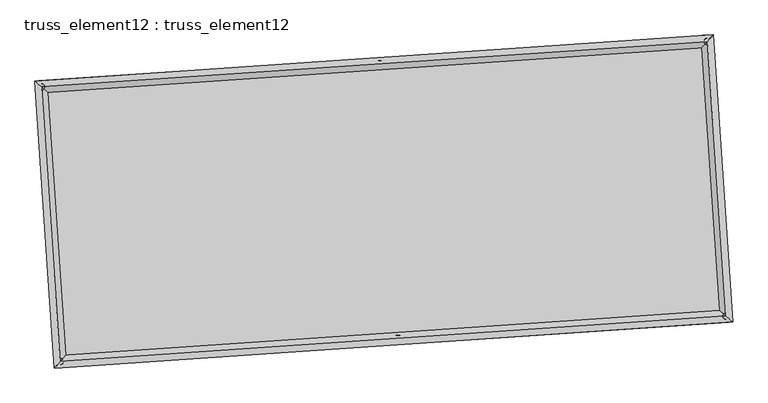
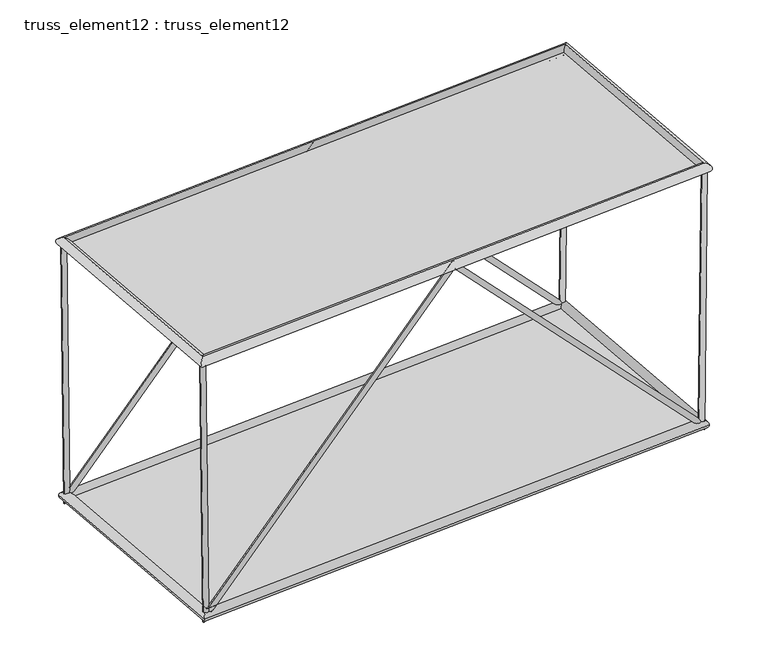
"""IFC4 building model written with IfcOpenShell, lengths in millimetres: plate geometry, truss_element12 : truss_element12."""

import ifcopenshell
import ifcopenshell.guid

model = None  # the IFC model being written
_history = None  # IfcOwnerHistory: only IFC2X3 demands one
_inside = {}  # id of a spatial element -> (the spatial element, [elements in it])
_under = {}  # id of a project, library or spatial element -> (it, [spatial elements below it])
_declared = {}  # id of a project -> (the project, [libraries it declares])
_typed = {}  # id of a type object -> (the type object, [elements of that type])
_made_of = {}  # id of a material, layer set ... -> (it, [elements and type objects made of it])


def new_model(schema):
    """Start an empty IFC model of exactly this schema.

    Asked for "IFC4X3", IfcOpenShell would pick the latest addendum, in which some entities
    have other attributes; the version numbers below select the first issue.
    IFC2X3 requires an IfcOwnerHistory on every rooted entity: one is made here for all.
    """
    global model, _history
    if schema == "IFC4X3":
        model = ifcopenshell.file(schema_version=(4, 3, 0, 0))
    else:
        model = ifcopenshell.file(schema=schema)
    _inside.clear()
    _under.clear()
    _declared.clear()
    _typed.clear()
    _made_of.clear()
    _history = None
    if model.schema == "IFC2X3":
        org = make("IfcOrganization", Name="unknown")
        user = make(
            "IfcPersonAndOrganization",
            ThePerson=make("IfcPerson", FamilyName="unknown"),
            TheOrganization=org,
        )
        app = make(
            "IfcApplication",
            ApplicationDeveloper=org,
            Version="unknown",
            ApplicationFullName="unknown",
            ApplicationIdentifier="unknown",
        )
        _history = make(
            "IfcOwnerHistory",
            OwningUser=user,
            OwningApplication=app,
            ChangeAction="ADDED",
            CreationDate=0,
        )
    return model


def make(cls, **values):
    """One entity of the class cls with the attributes given. An attribute that is None is left unset."""
    return model.create_entity(
        cls, **{name: value for name, value in values.items() if value is not None}
    )


def rooted(cls, **values):
    """An entity with a GlobalId (a new one), such as an element, a storey or a relation."""
    return make(cls, GlobalId=ifcopenshell.guid.new(), OwnerHistory=_history, **values)


def si_unit(unit_type, name, prefix=None):
    """IfcSIUnit, for example si_unit("LENGTHUNIT", "METRE", prefix="MILLI")."""
    return make("IfcSIUnit", UnitType=unit_type, Prefix=prefix, Name=name)


def assignment(units):
    """IfcUnitAssignment: the units of a project."""
    return None if units is None else make("IfcUnitAssignment", Units=units)


def point(xyz):
    """IfcCartesianPoint."""
    return None if xyz is None else make("IfcCartesianPoint", Coordinates=xyz)


def direction(xyz):
    """IfcDirection."""
    return None if xyz is None else make("IfcDirection", DirectionRatios=xyz)


def frame(location, z_axis=None, x_axis=None):
    """IfcAxis2Placement3D, a coordinate frame: its origin and axes. An axis left out is left unset."""
    return make(
        "IfcAxis2Placement3D",
        Location=point(location),
        Axis=direction(z_axis),
        RefDirection=direction(x_axis),
    )


def origin():
    """The frame at (0, 0, 0) with its axes left unset."""
    return frame((0.0, 0.0, 0.0))


def origin_with_axes():
    """The frame at (0, 0, 0) with the z axis (0, 0, 1) and the x axis (1, 0, 0) written out."""
    return frame((0.0, 0.0, 0.0), z_axis=(0.0, 0.0, 1.0), x_axis=(1.0, 0.0, 0.0))


def place(relative_to, where):
    """IfcLocalPlacement: puts the frame where relative to a parent placement (None: the world)."""
    return make(
        "IfcLocalPlacement", PlacementRelTo=relative_to, RelativePlacement=where
    )


def context(
    kind, dimensions, precision=None, world=None, true_north=None, identifier=None
):
    """IfcGeometricRepresentationContext, for example the 3D "Model" context."""
    return make(
        "IfcGeometricRepresentationContext",
        ContextIdentifier=identifier,
        ContextType=kind,
        CoordinateSpaceDimension=dimensions,
        Precision=precision,
        WorldCoordinateSystem=world,
        TrueNorth=true_north,
    )


def project(units=None, contexts=None):
    """IfcProject with its units and contexts."""
    return rooted(
        "IfcProject",
        Name="project",
        RepresentationContexts=contexts,
        UnitsInContext=assignment(units),
    )


def spatial(cls, under=None, at=None, **own):
    """A site, building, storey or space (cls), placed at a placement, below another one or the project."""
    s = rooted(cls, ObjectPlacement=at, **own)
    if under is not None:
        _under.setdefault(under.id(), (under, []))[1].append(s)
    return s


def polyline(points):
    """IfcPolyline through the points."""
    return make("IfcPolyline", Points=[point(p) for p in points])


def circle_curve(where, radius):
    """IfcCircle in the frame where."""
    return make("IfcCircle", Position=where, Radius=radius)


def ellipse_curve(where, semi_axis1, semi_axis2):
    """IfcEllipse in the frame where."""
    return make(
        "IfcEllipse", Position=where, SemiAxis1=semi_axis1, SemiAxis2=semi_axis2
    )


def outline(outer, holes=None, kind="AREA"):
    """IfcArbitraryClosedProfileDef: a profile drawn as a closed curve; with holes, ...WithVoids."""
    if holes is None:
        return make("IfcArbitraryClosedProfileDef", ProfileType=kind, OuterCurve=outer)
    return make(
        "IfcArbitraryProfileDefWithVoids",
        ProfileType=kind,
        OuterCurve=outer,
        InnerCurves=holes,
    )


def extrude(swept, where, along, depth):
    """IfcExtrudedAreaSolid: the profile swept, set in the frame where, extruded along a direction by depth."""
    return make(
        "IfcExtrudedAreaSolid",
        SweptArea=swept,
        Position=where,
        ExtrudedDirection=direction(along),
        Depth=depth,
    )


def shape(context_of_items, identifier, shape_type, items):
    """IfcShapeRepresentation: the items that make up one representation, for example the "Body"."""
    return make(
        "IfcShapeRepresentation",
        ContextOfItems=context_of_items,
        RepresentationIdentifier=identifier,
        RepresentationType=shape_type,
        Items=items,
    )


def source(mapping_origin, context_of_items, identifier, shape_type, items):
    """IfcRepresentationMap: a shape defined once, which mapped items show again and again."""
    return make(
        "IfcRepresentationMap",
        MappingOrigin=mapping_origin,
        MappedRepresentation=shape(context_of_items, identifier, shape_type, items),
    )


def transform(
    local_origin,
    x_axis=None,
    y_axis=None,
    z_axis=None,
    scale=None,
    scale2=None,
    scale3=None,
    uniform=True,
):
    """IfcCartesianTransformationOperator3D, or its non-uniform kind. x_axis, y_axis, z_axis: its Axis1, 2, 3."""
    if uniform:
        return make(
            "IfcCartesianTransformationOperator3D",
            Axis1=direction(x_axis),
            Axis2=direction(y_axis),
            LocalOrigin=point(local_origin),
            Scale=scale,
            Axis3=direction(z_axis),
        )
    return make(
        "IfcCartesianTransformationOperator3DnonUniform",
        Axis1=direction(x_axis),
        Axis2=direction(y_axis),
        LocalOrigin=point(local_origin),
        Scale=scale,
        Axis3=direction(z_axis),
        Scale2=scale2,
        Scale3=scale3,
    )


def mapped(mapping_source, mapping_target):
    """IfcMappedItem: shows the shape of a source again, moved by a transform."""
    return make(
        "IfcMappedItem", MappingSource=mapping_source, MappingTarget=mapping_target
    )


def made_of(thing, what):
    """Note that an element or type object is made of a material, layer set ...; save() writes the relation."""
    if what is not None:
        _made_of.setdefault(what.id(), (what, []))[1].append(thing)
    return thing


def element(
    cls,
    number,
    at=None,
    inside=None,
    cuts=None,
    type_object=None,
    material=None,
    context=None,
    identifier="Body",
    shape_type=None,
    held_by="IfcProductDefinitionShape",
    body=None,
    shapes=None,
    **own,
):
    """One element of the class cls, such as IfcWall. Its Tag is "e" and its number.

    at: its placement. inside: the storey or other place that contains it. cuts: it is an
    opening in that element (IfcRelVoidsElement). A single representation is given by context,
    identifier, shape_type and body (its items); several are given by shapes. held_by: the class
    of the entity that holds the representations. save() writes the other relations.
    """
    e = rooted(cls, Tag="e%d" % number, ObjectPlacement=at, **own)
    if body is not None:
        shapes = [shape(context, identifier, shape_type, body)]
    if shapes is not None:
        e.Representation = make(held_by, Representations=shapes)
    if inside is not None:
        _inside.setdefault(inside.id(), (inside, []))[1].append(e)
    if cuts is not None:
        rooted(
            "IfcRelVoidsElement", RelatingBuildingElement=cuts, RelatedOpeningElement=e
        )
    if type_object is not None:
        _typed.setdefault(type_object.id(), (type_object, []))[1].append(e)
    return made_of(e, material)


def aggregate(whole, parts):
    """IfcRelAggregates: a whole, such as a stair, and the parts it consists of."""
    return rooted("IfcRelAggregates", RelatingObject=whole, RelatedObjects=parts)


def save(model, path):
    """Write the relations noted so far, then the file.

    IfcRelAggregates (storeys below a building ...), IfcRelContainedInSpatialStructure (elements
    in a storey), IfcRelDefinesByType, IfcRelAssociatesMaterial and IfcRelDeclares: one each for
    every whole, place, type object, material and project.
    """
    for whole, parts in _under.values():
        aggregate(whole, parts)
    for where, things in _inside.values():
        rooted(
            "IfcRelContainedInSpatialStructure",
            RelatedElements=things,
            RelatingStructure=where,
        )
    for kind, things in _typed.values():
        rooted("IfcRelDefinesByType", RelatedObjects=things, RelatingType=kind)
    for what, things in _made_of.values():
        rooted("IfcRelAssociatesMaterial", RelatedObjects=things, RelatingMaterial=what)
    for by, libraries in _declared.values():
        rooted("IfcRelDeclares", RelatingContext=by, RelatedDefinitions=libraries)
    model.write(path)


def plane_surface(at):
    """IfcPlane: the flat surface through the origin of the frame at, square to its z axis."""
    return make("IfcPlane", Position=at)


def cylinder_surface(at, radius):
    """IfcCylindricalSurface: all points at the distance radius from the z axis of the frame at."""
    return make("IfcCylindricalSurface", Position=at, Radius=radius)


def advanced_brep(points, edges, surfaces, faces):
    """IfcAdvancedBrep: a solid bounded by faces that lie on surfaces and meet in shared edges.

    An edge is (start, end): straight between two places in points (the first is 0);
    or (start, end, curve); or (start, end, curve, False) where it runs against its curve.
    A face is (place in surfaces, loops), or (place, loops, False) where it looks against
    its surface's normal. A loop lists edges by number (the first is 1), with a minus sign
    where the edge is run from its end to its start. The first loop is the outer one.
    """
    corners = [point(p) for p in points]
    vertices = [make("IfcVertexPoint", VertexGeometry=c) for c in corners]
    made = []
    for start, end, *more in edges:
        made.append(
            make(
                "IfcEdgeCurve",
                EdgeStart=vertices[start],
                EdgeEnd=vertices[end],
                EdgeGeometry=more[0] if more else make("IfcPolyline", Points=[corners[start], corners[end]]),
                SameSense=more[1] if len(more) > 1 else True,
            )
        )
    hull = []
    for where, loops, *sense in faces:
        bounds = []
        for j, loop in enumerate(loops):
            ring = [make("IfcOrientedEdge", EdgeElement=made[abs(k) - 1], Orientation=k > 0) for k in loop]
            bounds.append(
                make(
                    "IfcFaceOuterBound" if j == 0 else "IfcFaceBound",
                    Bound=make("IfcEdgeLoop", EdgeList=ring),
                    Orientation=True,
                )
            )
        hull.append(make("IfcAdvancedFace", Bounds=bounds, FaceSurface=surfaces[where], SameSense=sense[0] if sense else True))
    return make("IfcAdvancedBrep", Outer=make("IfcClosedShell", CfsFaces=hull))


def truss_element12_truss_element12_1e288aef(model_context):
    return source(origin(), model_context, "Body", "SolidModel", [
        advanced_brep(
        [(-3721.8541699, 2272.3433372, 5000.243792), (-3820.9510531, 2258.982503, 4999.1054445), (-3666.3357635, 2276.1289263, 122.7527544), (-3762.6511193, 2262.9577538, -122.7527544), (1063.2103796, 2598.6186991, 5071.8018953), (1063.6661844, 2592.0459842, 4927.5587941), (5793.7499875, 2921.1762125, 122.759853), (5891.0109895, 2921.204276, -122.759853), (5848.2824161, 2924.8945715, 5000.2451385), (5948.275935, 2925.108955, 4999.1270036)],
        [
            (0, 1, circle_curve(frame((-3771.4026115, 2265.6629201, 4999.6746183), z_axis=(-0.011381834017515616, -0.0007760839952527173, 0.9999349236565499), x_axis=(-0.13360848187270624, 0.9910339089151396, -0.0007516329220677924)), 50.0)),
            (1, 0, circle_curve(frame((-3771.4026115, 2265.6629201, 4999.6746183), z_axis=(-0.011381834017515616, -0.0007760839952527173, 0.9999349236565499), x_axis=(-0.13360848187270624, 0.9910339089151396, -0.0007516329220677924)), 50.0)),
            (0, 2),
            (2, 3, ellipse_curve(frame((-3714.4934414, 2269.54334, 0.0), z_axis=(-0.9278994784854547, -0.06326993816178475, 0.36742274392234436), x_axis=(0.36657157095159426, 0.024995121954192616, 0.9300540453374608)), 132.271936, 50.0)),
            (3, 1),
            (3, 2, ellipse_curve(frame((-3714.4934414, 2269.54334, 0.0), z_axis=(-0.9278994784854547, -0.06326993816178475, 0.36742274392234436), x_axis=(0.36657157095159426, 0.024995121954192616, 0.9300540453374608)), 132.271936, 50.0)),
            (2, 4),
            (4, 5, ellipse_curve(frame((1063.438282, 2595.3323417, 4999.6803447), z_axis=(-0.9976833946832313, -0.06802823813381093, -5.281811364997211e-05), x_axis=(5.2695755000598474e-05, 3.593123218122507e-06, -0.9999999986051235)), 72.2785958, 50.0)),
            (5, 3),
            (5, 4, ellipse_curve(frame((1063.438282, 2595.3323417, 4999.6803447), z_axis=(-0.9976833946832313, -0.06802823813381093, -5.281811364997211e-05), x_axis=(5.2695755000598474e-05, 3.593123218122507e-06, -0.9999999986051235)), 72.2785958, 50.0)),
            (4, 6),
            (6, 7, ellipse_curve(frame((5842.3804885, 2921.1902443, 0.0), z_axis=(-0.9278429760300568, -0.06326608547413708, -0.3675660678850353), x_axis=(-0.3667145628894308, -0.025004872030870366, 0.9299974116843194)), 132.2876405, 50.0)),
            (7, 5),
            (7, 6, ellipse_curve(frame((5842.3804885, 2921.1902443, 0.0), z_axis=(-0.9278429760300568, -0.06326608547413708, -0.3675660678850353), x_axis=(-0.3667145628894308, -0.025004872030870366, 0.9299974116843194)), 132.2876405, 50.0)),
            (8, 9, circle_curve(frame((5898.2791756, 2925.0017632, 4999.6860711), z_axis=(0.011179737411862272, 0.0007623037959543959, 0.9999372142111346), x_axis=(-0.002152223979418104, 0.9999974114288641, -0.0007382868776594081)), 50.0)),
            (9, 8, circle_curve(frame((5898.2791756, 2925.0017632, 4999.6860711), z_axis=(0.011179737411862272, 0.0007623037959543959, 0.9999372142111346), x_axis=(-0.002152223979418104, 0.9999974114288641, -0.0007382868776594081)), 50.0)),
            (6, 8),
            (9, 7),
        ],
        [
            plane_surface(frame((-3771.4026115, 2315.662905, 4999.713425), z_axis=(-0.01138183401751662, -0.0007760839952526837, 0.99993492365655), x_axis=(0.9999352248292876, -8.833831430798961e-06, 0.01138183058939645))),
            cylinder_surface(frame((-3771.4026115, 2265.6629201, 4999.6746183), z_axis=(-0.011381834017515616, -0.0007760839952527173, 0.9999349236565499), x_axis=(-0.13360848187270624, 0.9910339089151396, -0.0007516329220677924)), 50.0),
            cylinder_surface(frame((-3714.4934414, 2269.54334, 0.0), z_axis=(-0.6901271226391988, -0.04705714507397151, -0.7221566171511742), x_axis=(-0.0204113902098155, 0.9987523882932022, -0.045574576556754245)), 50.0),
            cylinder_surface(frame((1063.438282, 2595.3323417, 4999.6803447), z_axis=(-0.690203227964863, -0.04706233440682505, 0.72208354141821), x_axis=(-0.11534466276751382, 0.9922792493126465, -0.04557960239601923)), 50.0),
            plane_surface(frame((5898.2791756, 2875.0017778, 4999.7241886), z_axis=(0.011179737411861788, 0.0007623037959489832, 0.9999372142111346), x_axis=(0.9999375047828748, -8.522888906625786e-06, -0.011179734163143003))),
            cylinder_surface(frame((5842.3804885, 2921.1902443, 0.0), z_axis=(-0.011179737411862274, -0.0007623037959543961, -0.9999372142111348), x_axis=(-0.002152223979418104, 0.9999974114288641, -0.0007382868776594081)), 50.0),
        ],
        [
            (0, [[1, 2]]),
            (1, [[-1, 3, 4, 5]]),
            (1, [[-2, -5, 6, -3]]),
            (2, [[-4, 7, 8, 9]]),
            (2, [[-6, -9, 10, -7]]),
            (3, [[-8, 11, 12, 13]]),
            (3, [[-10, -13, 14, -11]]),
            (4, [[15, 16]]),
            (5, [[-12, 17, -16, 18]]),
            (5, [[-14, -18, -15, -17]]),
        ],
    ),
        advanced_brep(
        [(-3449.741217, -1718.3902471, 5000.243792), (-3548.8381002, -1731.7510813, 4999.1054445), (-3394.2228106, -1714.604658, 122.7527544), (-3490.5381664, -1727.7758305, -122.7527544), (1335.3233326, -1392.1148852, 5071.8018953), (1335.7791373, -1398.6876001, 4927.5587941), (6065.8629405, -1069.5573718, 122.759853), (6163.1239424, -1069.5293083, -122.759853), (6120.395369, -1065.8390128, 5000.2451385), (6220.3888879, -1065.6246293, 4999.1270036)],
        [
            (0, 1, circle_curve(frame((-3499.2896586, -1725.0706642, 4999.6746183), z_axis=(-0.0113818340175155, -0.0007760839952527034, 0.9999349236565499), x_axis=(-0.1336084818727064, 0.9910339089151396, -0.0007516329220677924)), 50.0)),
            (1, 0, circle_curve(frame((-3499.2896586, -1725.0706642, 4999.6746183), z_axis=(-0.0113818340175155, -0.0007760839952527034, 0.9999349236565499), x_axis=(-0.1336084818727064, 0.9910339089151396, -0.0007516329220677924)), 50.0)),
            (0, 2),
            (2, 3, ellipse_curve(frame((-3442.3804885, -1721.1902443, 0.0), z_axis=(-0.927899478485455, -0.06326993816178478, 0.3674227439223443), x_axis=(0.36657157095159415, 0.02499512195419262, 0.9300540453374606)), 132.271936, 50.0)),
            (3, 1),
            (3, 2, ellipse_curve(frame((-3442.3804885, -1721.1902443, 0.0), z_axis=(-0.927899478485455, -0.06326993816178478, 0.3674227439223443), x_axis=(0.36657157095159415, 0.02499512195419262, 0.9300540453374606)), 132.271936, 50.0)),
            (2, 4),
            (4, 5, ellipse_curve(frame((1335.5512349, -1395.4012426, 4999.6803447), z_axis=(-0.9976833946832313, -0.06802823813381102, -5.281811365021285e-05), x_axis=(5.269575500075221e-05, 3.59312321818977e-06, -0.9999999986051235)), 72.2785958, 50.0)),
            (5, 3),
            (5, 4, ellipse_curve(frame((1335.5512349, -1395.4012426, 4999.6803447), z_axis=(-0.9976833946832313, -0.06802823813381102, -5.281811365021285e-05), x_axis=(5.269575500075221e-05, 3.59312321818977e-06, -0.9999999986051235)), 72.2785958, 50.0)),
            (4, 6),
            (6, 7, ellipse_curve(frame((6114.4934414, -1069.54334, 0.0), z_axis=(-0.9278429760300566, -0.06326608547413719, -0.36756606788503576), x_axis=(-0.3667145628894313, -0.025004872030870456, 0.9299974116843193)), 132.2876405, 50.0)),
            (7, 5),
            (7, 6, ellipse_curve(frame((6114.4934414, -1069.54334, 0.0), z_axis=(-0.9278429760300566, -0.06326608547413719, -0.36756606788503576), x_axis=(-0.3667145628894313, -0.025004872030870456, 0.9299974116843193)), 132.2876405, 50.0)),
            (8, 9, circle_curve(frame((6170.3921285, -1065.7318211, 4999.6860711), z_axis=(0.011179737411862045, 0.0007623037959543686, 0.9999372142111348), x_axis=(-0.0021522239794181794, 0.999997411428864, -0.0007382868776593801)), 50.0)),
            (9, 8, circle_curve(frame((6170.3921285, -1065.7318211, 4999.6860711), z_axis=(0.011179737411862045, 0.0007623037959543686, 0.9999372142111348), x_axis=(-0.0021522239794181794, 0.999997411428864, -0.0007382868776593801)), 50.0)),
            (6, 8),
            (9, 7),
        ],
        [
            plane_surface(frame((-3499.2896586, -1675.0706793, 4999.713425), z_axis=(-0.01138183401751662, -0.0007760839952526816, 0.99993492365655), x_axis=(0.9999352248292876, -8.833831430798961e-06, 0.01138183058939645))),
            cylinder_surface(frame((-3499.2896586, -1725.0706642, 4999.6746183), z_axis=(-0.0113818340175155, -0.0007760839952527034, 0.9999349236565499), x_axis=(-0.1336084818727064, 0.9910339089151396, -0.0007516329220677924)), 50.0),
            cylinder_surface(frame((-3442.3804885, -1721.1902443, 0.0), z_axis=(-0.6901271226391986, -0.04705714507397152, -0.7221566171511744), x_axis=(-0.020411390209815434, 0.9987523882932022, -0.045574576556754315)), 50.0),
            cylinder_surface(frame((1335.5512349, -1395.4012426, 4999.6803447), z_axis=(-0.6902032279648631, -0.047062334406825154, 0.7220835414182099), x_axis=(-0.11534466276751408, 0.9922792493126465, -0.04557960239601936)), 50.0),
            plane_surface(frame((6170.3921285, -1115.7318065, 4999.7241886), z_axis=(0.011179737411861788, 0.0007623037959489812, 0.9999372142111346), x_axis=(0.9999375047828748, -8.522888906625786e-06, -0.011179734163143003))),
            cylinder_surface(frame((6114.4934414, -1069.54334, 0.0), z_axis=(-0.011179737411862043, -0.0007623037959543684, -0.9999372142111346), x_axis=(-0.0021522239794181794, 0.999997411428864, -0.0007382868776593801)), 50.0),
        ],
        [
            (0, [[1, 2]]),
            (1, [[-1, 3, 4, 5]]),
            (1, [[-2, -5, 6, -3]]),
            (2, [[-4, 7, 8, 9]]),
            (2, [[-6, -9, 10, -7]]),
            (3, [[-8, 11, 12, 13]]),
            (3, [[-10, -13, 14, -11]]),
            (4, [[15, 16]]),
            (5, [[-12, 17, -16, 18]]),
            (5, [[-14, -18, -15, -17]]),
        ],
    ),
        advanced_brep(
        [(-3499.2866492, -1725.0673288, 4909.6746183), (-3499.292668, -1725.0739997, 5089.6746182), (-3771.4060458, 2265.6658161, 5089.6746182), (-3771.3991772, 2265.660024, 4909.6746183), (5898.2819728, 2925.0050842, 5089.686071), (5898.2763784, 2924.9984423, 4909.6860711), (6170.3953506, -1065.7347316, 5089.686071), (6170.3889064, -1065.7289105, 4909.6860711)],
        [
            (0, 1, ellipse_curve(frame((-3499.2896586, -1725.0706642, 4999.6746183), z_axis=(-0.7535719234049658, 0.657365466278114, -8.3555725473804e-07), x_axis=(-0.6573654662775879, -0.7535719234054246, -8.355572547380254e-07)), 127.2792206, 90.0)),
            (1, 2),
            (2, 3, ellipse_curve(frame((-3771.4026115, 2265.6629201, 4999.6746183), z_axis=(-0.6573654662775877, -0.7535719234054249, -8.355572547380119e-07), x_axis=(0.7535719234049659, -0.6573654662781139, 8.355572547380267e-07)), 127.2792206, 90.0)),
            (3, 0),
            (1, 0, ellipse_curve(frame((-3499.2896586, -1725.0706642, 4999.6746183), z_axis=(-0.7535719234049658, 0.657365466278114, -8.3555725473804e-07), x_axis=(-0.6573654662775879, -0.7535719234054246, -8.355572547380254e-07)), 127.2792206, 90.0)),
            (3, 2, ellipse_curve(frame((-3771.4026115, 2265.6629201, 4999.6746183), z_axis=(-0.6573654662775877, -0.7535719234054249, -8.355572547380119e-07), x_axis=(0.7535719234049659, -0.6573654662781139, 8.355572547380267e-07)), 127.2792206, 90.0)),
            (2, 4),
            (4, 5, ellipse_curve(frame((5898.2791756, 2925.0017632, 4999.6860711), z_axis=(-0.7535719234049658, 0.657365466278114, -8.355572547380136e-07), x_axis=(-0.6573654662775879, -0.7535719234054248, -8.355572547380251e-07)), 127.2792206, 90.0)),
            (5, 3),
            (5, 4, ellipse_curve(frame((5898.2791756, 2925.0017632, 4999.6860711), z_axis=(-0.7535719234049658, 0.657365466278114, -8.355572547380136e-07), x_axis=(-0.6573654662775879, -0.7535719234054248, -8.355572547380251e-07)), 127.2792206, 90.0)),
            (4, 6),
            (6, 7, ellipse_curve(frame((6170.3921285, -1065.7318211, 4999.6860711), z_axis=(0.6573654662775877, 0.7535719234054248, 8.355572547380384e-07), x_axis=(-0.7535719234049659, 0.657365466278114, -8.355572547380273e-07)), 127.2792206, 90.0)),
            (7, 5),
            (7, 6, ellipse_curve(frame((6170.3921285, -1065.7318211, 4999.6860711), z_axis=(0.6573654662775877, 0.7535719234054248, 8.355572547380384e-07), x_axis=(-0.7535719234049659, 0.657365466278114, -8.355572547380273e-07)), 127.2792206, 90.0)),
            (6, 1),
            (0, 7),
        ],
        [
            cylinder_surface(frame((-3499.2896586, -1725.0706642, 4999.6746183), z_axis=(0.06802823822870131, -0.9976833960748765, 0.0), x_axis=(-0.9976833954326236, -0.06802823818490852, -3.58815903472379e-05)), 90.0),
            cylinder_surface(frame((-3771.4026115, 2265.6629201, 4999.6746183), z_axis=(-0.99768339607418, -0.06802823822865506, -1.1816564017897381e-06), x_axis=(-0.06802823814683823, 0.9976833954770179, -3.4699933946159566e-05)), 90.0),
            cylinder_surface(frame((5898.2791756, 2925.0017632, 4999.6860711), z_axis=(-0.06802823822870106, 0.9976833960748765, 0.0), x_axis=(0.9976833955144404, 0.06802823819048705, -3.351827754508122e-05)), 90.0),
            cylinder_surface(frame((6170.3921285, -1065.7318211, 4999.6860711), z_axis=(0.99768339607418, 0.06802823822865493, 1.181656401789757e-06), x_axis=(0.06802823822865493, -0.9976833954714391, -3.469993394615955e-05)), 90.0),
        ],
        [
            (0, [[1, 2, 3, 4]]),
            (0, [[5, -4, 6, -2]]),
            (1, [[-3, 7, 8, 9]]),
            (1, [[-6, -9, 10, -7]]),
            (2, [[-8, 11, 12, 13]]),
            (2, [[-10, -13, 14, -11]]),
            (3, [[-12, 15, -1, 16]]),
            (3, [[-14, -16, -5, -15]]),
        ],
    ),
        advanced_brep(
        [(-3358.7115243, -1625.2761972, 0.0), (-3526.0494527, -1817.1042913, 0.0), (-3810.4074885, 2353.2123043, 0.0), (-3618.5793943, 2185.8743758, 0.0), (5926.0494527, 3017.1042913, 0.0), (5758.7115243, 2825.2761972, 0.0), (6210.4074885, -1153.2123043, 0.0), (6018.5793943, -985.8743758, 0.0)],
        [
            (0, 1, ellipse_curve(frame((-3442.3804885, -1721.1902443, 0.0), z_axis=(-0.7535719234054579, 0.6573654662780809, 0.0), x_axis=(-0.657365466278081, -0.7535719234054578, 0.0)), 127.2792206, 90.0)),
            (1, 2),
            (2, 3, ellipse_curve(frame((-3714.4934414, 2269.54334, 0.0), z_axis=(-0.6573654662780808, -0.7535719234054579, 0.0), x_axis=(0.7535719234054578, -0.6573654662780809, 0.0)), 127.2792206, 90.0)),
            (3, 0),
            (1, 0, ellipse_curve(frame((-3442.3804885, -1721.1902443, 0.0), z_axis=(-0.7535719234054579, 0.6573654662780809, 0.0), x_axis=(-0.657365466278081, -0.7535719234054578, 0.0)), 127.2792206, 90.0)),
            (3, 2, ellipse_curve(frame((-3714.4934414, 2269.54334, 0.0), z_axis=(-0.6573654662780808, -0.7535719234054579, 0.0), x_axis=(0.7535719234054578, -0.6573654662780809, 0.0)), 127.2792206, 90.0)),
            (2, 4),
            (4, 5, ellipse_curve(frame((5842.3804885, 2921.1902443, 0.0), z_axis=(-0.7535719234054579, 0.6573654662780809, 0.0), x_axis=(-0.6573654662780809, -0.7535719234054578, 0.0)), 127.2792206, 90.0)),
            (5, 3),
            (5, 4, ellipse_curve(frame((5842.3804885, 2921.1902443, 0.0), z_axis=(-0.7535719234054579, 0.6573654662780809, 0.0), x_axis=(-0.6573654662780809, -0.7535719234054578, 0.0)), 127.2792206, 90.0)),
            (4, 6),
            (6, 7, ellipse_curve(frame((6114.4934414, -1069.54334, 0.0), z_axis=(0.6573654662780809, 0.7535719234054579, 0.0), x_axis=(-0.7535719234054578, 0.6573654662780809, 0.0)), 127.2792206, 90.0)),
            (7, 5),
            (7, 6, ellipse_curve(frame((6114.4934414, -1069.54334, 0.0), z_axis=(0.6573654662780809, 0.7535719234054579, 0.0), x_axis=(-0.7535719234054578, 0.6573654662780809, 0.0)), 127.2792206, 90.0)),
            (6, 1),
            (0, 7),
        ],
        [
            cylinder_surface(frame((-3442.3804885, -1721.1902443, 0.0), z_axis=(0.06802823822870059, -0.9976833960748767, 0.0), x_axis=(-0.9976833960748767, -0.06802823822870059, 0.0)), 90.0),
            cylinder_surface(frame((-3714.4934414, 2269.54334, 0.0), z_axis=(-0.9976833960748767, -0.06802823822870172, 0.0), x_axis=(-0.06802823822870172, 0.9976833960748767, 0.0)), 90.0),
            cylinder_surface(frame((5842.3804885, 2921.1902443, 0.0), z_axis=(-0.06802823822870048, 0.9976833960748768, 0.0), x_axis=(0.9976833960748768, 0.06802823822870048, 0.0)), 90.0),
            cylinder_surface(frame((6114.4934414, -1069.54334, 0.0), z_axis=(0.9976833960748767, 0.06802823822870152, 0.0), x_axis=(0.06802823822870152, -0.9976833960748767, 0.0)), 90.0),
        ],
        [
            (0, [[1, 2, 3, 4]]),
            (0, [[5, -4, 6, -2]]),
            (1, [[-3, 7, 8, 9]]),
            (1, [[-6, -9, 10, -7]]),
            (2, [[-8, 11, 12, 13]]),
            (2, [[-10, -13, 14, -11]]),
            (3, [[-12, 15, -1, 16]]),
            (3, [[-14, -16, -5, -15]]),
        ],
    ),
        extrude(outline(polyline([(-3442.3804885, -1721.1902443), (-3714.4934414, 2269.54334), (5842.3804885, 2921.1902443), (6114.4934414, -1069.54334), (-3442.3804885, -1721.1902443)])), origin_with_axes(), (0.0, 0.0, 1.0), 20.0),
        extrude(outline(polyline([(-2000.0, 4846.0673121), (2000.0, 4846.0673121), (2000.0, -4846.0673121), (-2000.0, -4846.0673121), (-2000.0, 4846.0673121)])), frame((1199.4947585, 599.9655495, 4999.6803447), z_axis=(-1.1789189719312138e-06, -8.038600320542223e-08, 0.9999999999993019), x_axis=(-0.06802823822870074, 0.9976833960748767, 0.0)), (0.0, 0.0, 1.0), 20.0),
    ])


if __name__ == "__main__":
    model = new_model("IFC4")
    model_context = context("Model", 3, world=origin())
    ifc_project = project(units=[si_unit("LENGTHUNIT", "METRE", prefix="MILLI")], contexts=[model_context])
    site = spatial("IfcSite", under=ifc_project)
    building = spatial("IfcBuilding", under=site)
    placement = place(None, origin())
    truss_element12_truss_element12_shape = truss_element12_truss_element12_1e288aef(model_context)
    element("IfcPlate", 1, ObjectType="truss_element12 : truss_element12", at=placement, inside=building, context=model_context, shape_type="MappedRepresentation", body=[
        mapped(truss_element12_truss_element12_shape, transform((0.0, 0.0, 0.0), x_axis=(1.0, 0.0, 0.0), y_axis=(0.0, 1.0, 0.0), z_axis=(0.0, 0.0, 1.0))),
    ])
    save(model, "model.ifc")

# Revit data of these elements
# Type "truss_element12 : truss_element12"
#   steellbar1 = 90 mm
#   steelbar2 = 50 mm
#   offset1 = 5000 mm
#   M = Default Roof
# Element 1 (IfcPlate, "truss_element12 : truss_element12")
#   Materials on its faces: "Default Roof"
# Materials
#   "Default Roof": class "Miscellaneous", colour RGB 0 127 0, transparency 0, Comments = "Rendering appearance not upgraded Rendering appearance not upgraded ", Cost = 0
